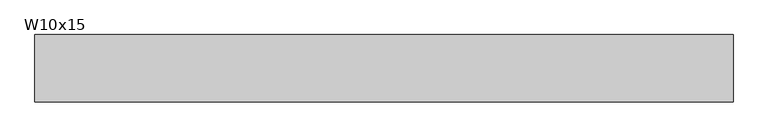
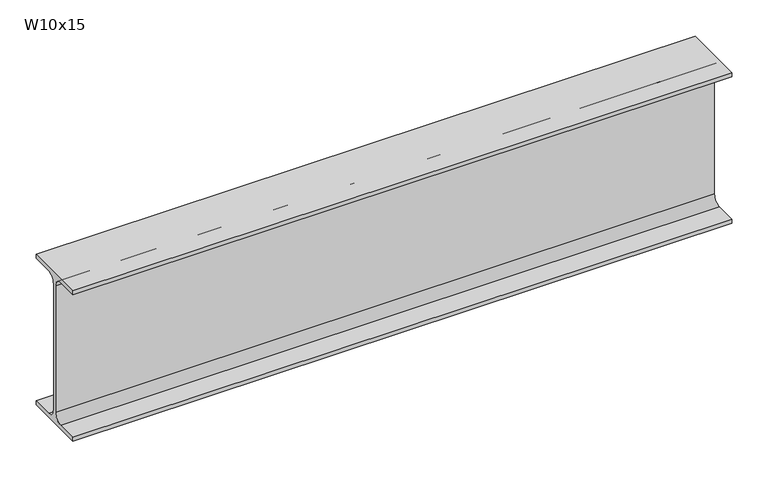
"""IFC4 building model written with IfcOpenShell, lengths in millimetres: beam geometry, RME W-Wide Flange : W10x15."""

from ifc_helpers import new_model, si_unit, point, frame, frame_2d, origin, place, context, project, spatial, polyline, circle_curve, trimmed, segment, composite_curve, outline, extrude, source, transform, mapped, element, save


def w10x15_ed4b60ef(model_context):
    return source(origin(), model_context, "Body", "SweptSolid", [
        extrude(outline(composite_curve([segment(polyline([(50.8, -120.142), (50.8, -127.0), (-50.8, -127.0), (-50.8, -120.142), (-16.7005, -120.142)]), True, "CONTINUOUS"), segment(trimmed(circle_curve(frame_2d((-16.7005, -106.3625)), 13.7795), [point((-16.7005, -120.142))], [point((-2.921, -106.3625))], True, "CARTESIAN"), True, "CONTINUOUS"), segment(polyline([(-2.921, -106.3625), (-2.921, 106.3625)]), True, "CONTINUOUS"), segment(trimmed(circle_curve(frame_2d((-16.7005, 106.3625)), 13.7795), [point((-2.921, 106.3625))], [point((-16.7005, 120.142))], True, "CARTESIAN"), True, "CONTINUOUS"), segment(polyline([(-16.7005, 120.142), (-50.8, 120.142), (-50.8, 127.0), (50.8, 127.0), (50.8, 120.142), (16.7005, 120.142)]), True, "CONTINUOUS"), segment(trimmed(circle_curve(frame_2d((16.7005, 106.3625)), 13.7795), [point((16.7005, 120.142))], [point((2.921, 106.3625))], True, "CARTESIAN"), True, "CONTINUOUS"), segment(polyline([(2.921, 106.3625), (2.921, -106.3625)]), True, "CONTINUOUS"), segment(trimmed(circle_curve(frame_2d((16.7005, -106.3625)), 13.7795), [point((2.921, -106.3625))], [point((16.7005, -120.142))], True, "CARTESIAN"), True, "CONTINUOUS"), segment(polyline([(16.7005, -120.142), (50.8, -120.142)]), True, "CONTINUOUS")], self_intersect=False)), frame((-519.1893433, 0.0, 0.0), z_axis=(1.0, 0.0, 0.0), x_axis=(0.0, 1.0, 0.0)), (0.0, 0.0, 1.0), 1051.0786871),
    ])


if __name__ == "__main__":
    model = new_model("IFC4")
    model_context = context("Model", 3, world=origin())
    ifc_project = project(units=[si_unit("LENGTHUNIT", "METRE", prefix="MILLI")], contexts=[model_context])
    site = spatial("IfcSite", under=ifc_project)
    building = spatial("IfcBuilding", under=site)
    placement = place(None, origin())
    w10x15_shape = w10x15_ed4b60ef(model_context)
    element("IfcBeam", 1, ObjectType="RME W-Wide Flange : W10x15", at=placement, inside=building, context=model_context, shape_type="MappedRepresentation", body=[
        mapped(w10x15_shape, transform((0.0, 0.0, 0.0), x_axis=(1.0, 0.0, 0.0), y_axis=(0.0, 1.0, 0.0), z_axis=(0.0, 0.0, 1.0))),
    ])
    save(model, "model.ifc")

# Revit data of these elements
# Type "RME W-Wide Flange : W10x15"
#   WELD P [instance default] = ""
#   WELD LE [instance default] = ""
#   WELD D [instance default] = ""
#   TOP SECTION SIZE [instance default] = ""
#   TOP SECTION LENGTH [instance default] = ""
#   REMARKS [instance default] = ""
#   REINF TYPE [instance default] = ""
#   Nominal Size = "W24"
#   End Bearing Capacity [instance default] = ""
#   BOT SECTION SIZE [instance default] = ""
#   BOT SECTION LENGTH [instance default] = ""
#   Assembly Code = "B10"
#   W = 15
#   Start Extension Calculation [instance default] = 10' - 0"
#   Start Extension [instance default] = -0' - 0 1/2"
#   End Extension Calculation [instance default] = 10' - 0"
#   End Extension [instance default] = -0' - 0 1/2"
#   Length [instance default] = 5' - 0"
#   bf = 0' - 4"
#   d = 0' - 10"
#   k = 0' - 0 13/16"
#   k2 = 0' - 0.5425"
#   tf = 0' - 0.27"
#   tw = 0' - 0.23"
#   A = 0.030625 SF
#   Structural Material [instance default] = Metal - Steel - ASTM A992
# Element 1 (IfcBeam, "RME W-Wide Flange : W10x15")
#   Materials on its faces: "Metal - Steel - ASTM A992"
# Materials
#   "Metal - Steel - ASTM A992": class "Metal", colour RGB 255 128 0, transparency 0
